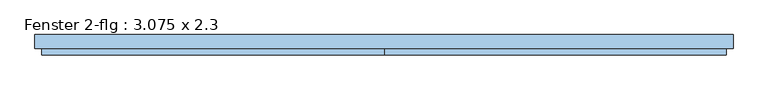
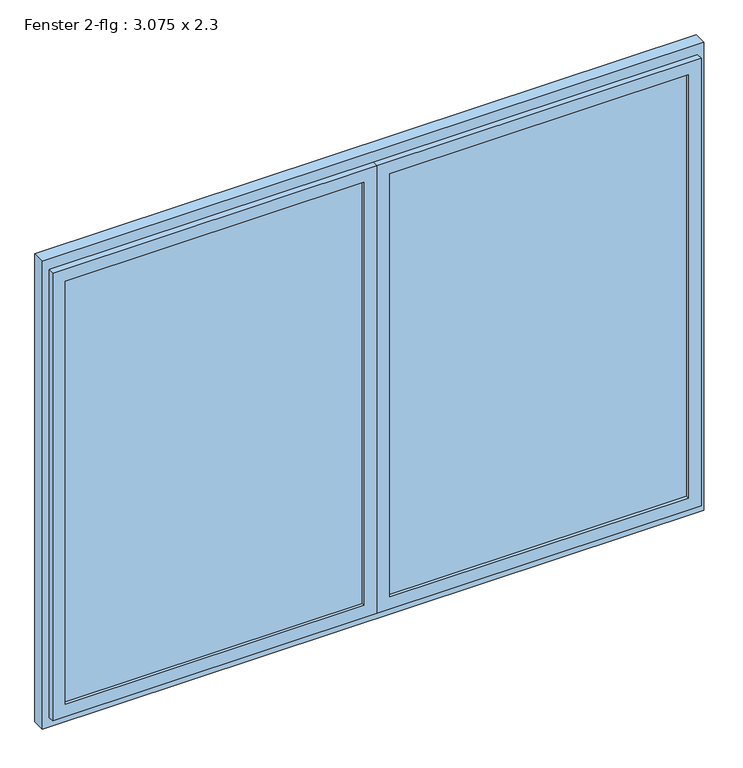
"""IFC4 building model written with IfcOpenShell, lengths in millimetres: window geometry, Fenster 2-flg : 3.075 x 2.3."""

from ifc_helpers import new_model, si_unit, frame, origin, place, context, project, spatial, polyline, outline, extrude, faceted_brep, source, transform, mapped, element, save


def fenster_2_flg_3_075_x_2_3_01af11f5(model_context):
    return source(origin(), model_context, "Body", "SolidModel", [
        extrude(outline(polyline([(30.0, -55.0), (-30.0, -55.0), (-30.0, 5.0), (30.0, 5.0), (30.0, -55.0)])), frame((0.0, 0.0, 1080.0), z_axis=(0.0, 0.0, 1.0), x_axis=(1.0, 0.0, 0.0)), (0.0, 0.0, 1.0), 2140.0),
        extrude(outline(polyline([(3300.0, -1537.5), (1000.0, -1537.5), (1000.0, 1537.5), (3300.0, 1537.5), (3300.0, -1537.5)]), holes=[polyline([(3220.0, -1477.5), (3220.0, 1477.5), (1080.0, 1477.5), (1080.0, -1477.5), (3220.0, -1477.5)])]), frame((0.0, -55.0, 0.0), z_axis=(0.0, 1.0, 0.0), x_axis=(0.0, 0.0, 1.0)), (0.0, 0.0, 1.0), 60.0),
        faceted_brep([(-1477.5, -55.0, 1080.0), (-1477.5, -25.0, 1080.0), (-30.0, -25.0, 1080.0), (-30.0, -55.0, 1080.0), (-30.0, -25.0, 3220.0), (-30.0, -55.0, 3220.0), (-1477.5, -25.0, 3220.0), (-60.0, -25.0, 3190.0), (-1447.5, -25.0, 3190.0), (-1447.5, -25.0, 1110.0), (-60.0, -25.0, 1110.0), (0.0, -55.0, 1050.0), (-1507.5, -55.0, 1050.0), (-1507.5, -55.0, 3250.0), (0.0, -55.0, 3250.0), (-1477.5, -55.0, 3220.0), (-1507.5, -85.0, 1050.0), (0.0, -85.0, 1050.0), (0.0, -85.0, 3250.0), (-1507.5, -85.0, 3250.0), (-60.0, -85.0, 1110.0), (-1447.5, -85.0, 1110.0), (-1447.5, -85.0, 3190.0), (-60.0, -85.0, 3190.0)], [[[0, 1, 2, 3]], [[3, 2, 4, 5]], [[2, 1, 6, 4], [7, 8, 9, 10]], [[11, 12, 13, 14], [5, 15, 0, 3]], [[16, 12, 11, 17]], [[17, 11, 14, 18]], [[18, 19, 16, 17], [20, 21, 22, 23]], [[9, 21, 20, 10]], [[10, 20, 23, 7]], [[15, 6, 1, 0]], [[19, 13, 12, 16]], [[8, 22, 21, 9]], [[5, 4, 6, 15]], [[18, 14, 13, 19]], [[7, 23, 22, 8]]]),
        faceted_brep([(30.0, -55.0, 1080.0), (30.0, -25.0, 1080.0), (1477.5, -25.0, 1080.0), (1477.5, -55.0, 1080.0), (1477.5, -25.0, 3220.0), (1477.5, -55.0, 3220.0), (30.0, -25.0, 3220.0), (1447.5, -25.0, 3190.0), (60.0, -25.0, 3190.0), (60.0, -25.0, 1110.0), (1447.5, -25.0, 1110.0), (1507.5, -55.0, 1050.0), (0.0, -55.0, 1050.0), (0.0, -55.0, 3250.0), (1507.5, -55.0, 3250.0), (30.0, -55.0, 3220.0), (0.0, -85.0, 1050.0), (1507.5, -85.0, 1050.0), (1507.5, -85.0, 3250.0), (0.0, -85.0, 3250.0), (1447.5, -85.0, 1110.0), (60.0, -85.0, 1110.0), (60.0, -85.0, 3190.0), (1447.5, -85.0, 3190.0)], [[[0, 1, 2, 3]], [[3, 2, 4, 5]], [[2, 1, 6, 4], [7, 8, 9, 10]], [[11, 12, 13, 14], [5, 15, 0, 3]], [[16, 12, 11, 17]], [[17, 11, 14, 18]], [[18, 19, 16, 17], [20, 21, 22, 23]], [[9, 21, 20, 10]], [[10, 20, 23, 7]], [[15, 6, 1, 0]], [[19, 13, 12, 16]], [[8, 22, 21, 9]], [[5, 4, 6, 15]], [[18, 14, 13, 19]], [[7, 23, 22, 8]]]),
        extrude(outline(polyline([(60.0, -40.0), (1447.5, -40.0), (1447.5, -70.0), (60.0, -70.0), (60.0, -40.0)])), frame((0.0, 0.0, 1110.0), z_axis=(0.0, 0.0, 1.0), x_axis=(1.0, 0.0, 0.0)), (0.0, 0.0, 1.0), 2080.0),
        extrude(outline(polyline([(-1447.5, -40.0), (-60.0, -40.0), (-60.0, -70.0), (-1447.5, -70.0), (-1447.5, -40.0)])), frame((0.0, 0.0, 1110.0), z_axis=(0.0, 0.0, 1.0), x_axis=(1.0, 0.0, 0.0)), (0.0, 0.0, 1.0), 2080.0),
    ])


if __name__ == "__main__":
    model = new_model("IFC4")
    model_context = context("Model", 3, world=origin())
    ifc_project = project(units=[si_unit("LENGTHUNIT", "METRE", prefix="MILLI")], contexts=[model_context])
    site = spatial("IfcSite", under=ifc_project)
    building = spatial("IfcBuilding", under=site)
    placement = place(None, origin())
    fenster_2_flg_3_075_x_2_3_shape = fenster_2_flg_3_075_x_2_3_01af11f5(model_context)
    element("IfcWindow", 1, ObjectType="Fenster 2-flg : 3.075 x 2.3", at=placement, inside=building, context=model_context, shape_type="MappedRepresentation", body=[
        mapped(fenster_2_flg_3_075_x_2_3_shape, transform((0.0, 0.0, 0.0), x_axis=(1.0, 0.0, 0.0), y_axis=(0.0, 1.0, 0.0), z_axis=(0.0, 0.0, 1.0))),
    ])
    save(model, "model.ifc")

# Revit data of these elements
# Project information
#   Projektausgabedatum = "Projekt Datum"
#   Projektstatus = "Projektstatus"
#   Kundenname = "Bauherr"
#   Projektadresse = "Projektadresse"
#   Projektname = "Projektname"
#   Projektnummer = "Projektnummer"
#   Verfasser Firma 1 = "Firma 1"
#   Verfasser Firma 2 = "Firma 2"
#   Verfasser PLZ Ort = "PLZ Ort"
#   Verfasser Strasse = "Strasse"
#   Verfasser Telefon = "Telefon"
#   Verfasser Telefax = "Telefax"
#   Verfasser eMail = "E-Mail"
# Type "Fenster 2-flg : 3.075 x 2.3"
#   Type Mark = "73"
#   Operation = "DoublePanelVertical"
#   Keynote = "16.05.01"
#   Visual Light Transmittance = 0.9
#   Solar Heat Gain Coefficient = 0.78
#   Rough Width = 3.075 m
#   Rough Height = 2.300 m
#   Heat Transfer Coefficient (U) = 3.6886 W/(m²·K)
#   Rahmentiefe = 0.060 m
#   Rahmenhöhe unten = 0.080 m
#   Höhe oberer  Rahmen = 0.080 m
#   Rahmenbreite = 0.060 m
#   Height = 2.300 m
#   Tiefe Flügel = 0.060 m
#   Flügelbreite = 0.060 m
#   Einbautiefe (von außen) [instance default] = 0.140 m
#   Width = 3.075 m
#   Öffnungsrichtung oben [instance default] = yes
#   Öffnungsrichtung in Draufsicht anzeigen [instance default] = no
#   Drehflügel 1 [instance default] = yes
#   Bild [instance default] = none
#   Glas [instance default] = none
#   Fensterflügel [instance default] = none
#   Äußere Fensterbank [instance default] = none
#   Innere Fensterbank [instance default] = none
#   Construction Type Id = ""
#   Wall Closure = (empty or 0)
#   Analytic Construction = (empty or 0)
# Element 1 (IfcWindow, "Fenster 2-flg : 3.075 x 2.3")
#   Einbautiefe (von außen) = 0.220 m
#   Materials on its faces: "Kunststoff - Weiß", "Glas"
# Materials
#   "Kunststoff - Weiß": class "Kunststoff", colour RGB 249 249 249, transparency 0, Cost = 0
#   "Glas": class "Glas", colour RGB 0 0 255, transparency 0.75, Comments = "Render-Darstellung nicht aktualisiert ", Cost = 0
